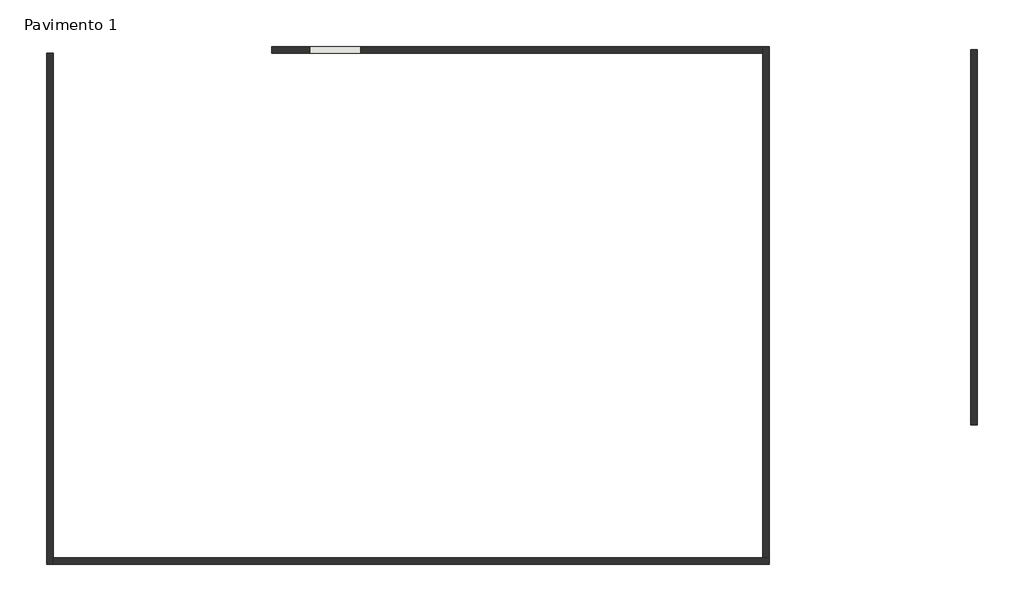
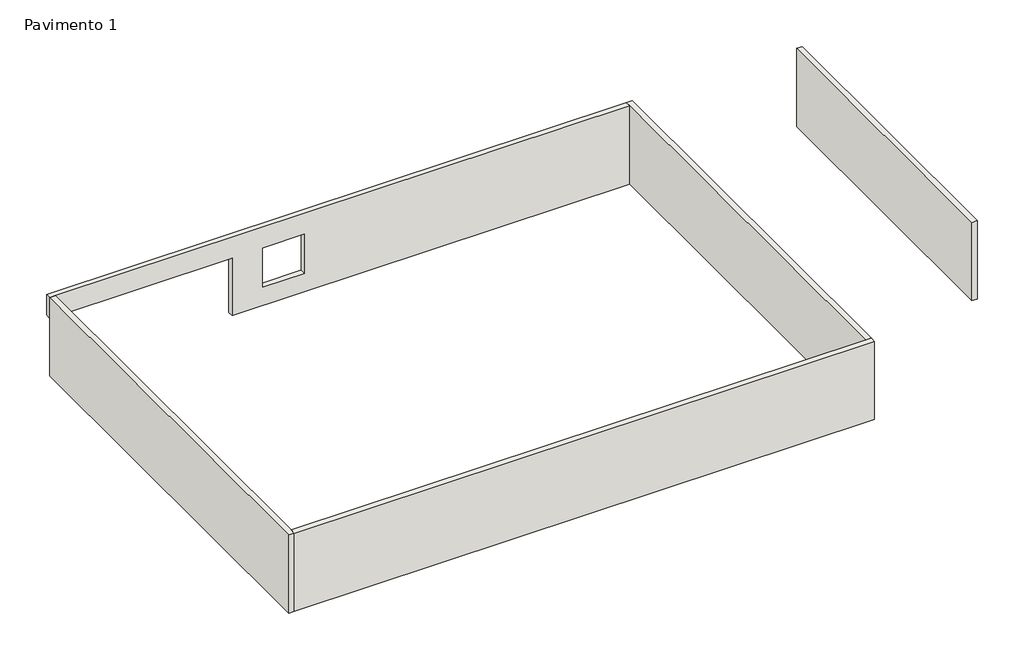
# One storey: 5 walls.
"""IFC4 building model written with IfcOpenShell, lengths in millimetres."""

from ifc_helpers import new_model, si_unit, origin, origin_with_axes, place, context, project, spatial, polyline, outline, extrude, faceted_brep, element, save

model = new_model("IFC4")

# Units and contexts
model_context = context("Model", 3, world=origin())
ifc_project = project(units=[si_unit("LENGTHUNIT", "METRE", prefix="MILLI")], contexts=[model_context])

# Site, building, storey
site = spatial("IfcSite", under=ifc_project)
building = spatial("IfcBuilding", under=site)
storey = spatial("IfcBuildingStorey", under=building, Name="Pavimento 1", Elevation=0.0)

# Walls
placement = place(None, origin())
element("IfcWall", 1, ObjectType=".Parede 020 cm", at=placement, inside=storey, context=model_context, shape_type="Brep", body=[
    faceted_brep([(-10926.104315, 4821.8769454, 2202.2712247), (-4326.104315, 4821.8769454, 2202.2712247), (-4326.104315, 4821.8769454, 0.0), (10073.895685, 4821.8769454, 0.0), (10073.895685, 4821.8769454, 3000.0), (-10726.104315, 4821.8769454, 3000.0), (-10926.104315, 4821.8769454, 3000.0), (-3207.6515293, 4821.8769454, 2202.2712247), (-1707.6515293, 4821.8769454, 2202.2712247), (-1707.6515293, 4821.8769454, 702.2712247), (-3207.6515293, 4821.8769454, 702.2712247), (-10926.104315, 5021.8769454, 2202.2712247), (-10926.104315, 5021.8769454, 3000.0), (10073.895685, 5021.8769454, 3000.0), (10073.895685, 5021.8769454, 0.0), (-4326.104315, 5021.8769454, 0.0), (-4326.104315, 5021.8769454, 2202.2712247), (-3207.6515293, 5021.8769454, 2202.2712247), (-3207.6515293, 5021.8769454, 702.2712247), (-1707.6515293, 5021.8769454, 702.2712247), (-1707.6515293, 5021.8769454, 2202.2712247)], [[[0, 1, 2, 3, 4, 5, 6], [7, 8, 9, 10]], [[11, 12, 13, 14, 15, 16], [17, 18, 19, 20]], [[0, 6, 12, 11]], [[4, 3, 14, 13]], [[3, 2, 15, 14]], [[6, 5, 4, 13, 12]], [[8, 7, 17, 20]], [[9, 8, 20, 19]], [[10, 9, 19, 18]], [[7, 10, 18, 17]], [[1, 0, 11, 16]], [[2, 1, 16, 15]]]),
])
element("IfcWall", 2, ObjectType=".Parede 020 cm", at=placement, inside=storey, context=model_context, shape_type="Brep", body=[
    faceted_brep([(-10726.104315, -10178.1230546, 0.0), (-10726.104315, -9978.1230546, 0.0), (-10726.104315, 4821.8769454, 0.0), (-10726.104315, 4821.8769454, 3000.0), (-10726.104315, -9978.1230546, 3000.0), (-10726.104315, -10178.1230546, 3000.0), (-10926.104315, -10178.1230546, 0.0), (-10926.104315, -10178.1230546, 3000.0), (-10926.104315, 4821.8769454, 3000.0), (-10926.104315, 4821.8769454, 2202.2712247), (-10926.104315, 4821.8769454, 0.0)], [[[0, 1, 2, 3, 4, 5]], [[6, 7, 8, 9, 10]], [[2, 1, 0, 6, 10]], [[5, 4, 3, 8, 7]], [[0, 5, 7, 6]], [[3, 2, 10, 9, 8]]]),
])
element("IfcWall", 3, ObjectType=".Parede 020 cm", at=placement, inside=storey, context=model_context, shape_type="Brep", body=[
    faceted_brep([(10273.895685, -9978.1230546, 0.0), (10073.895685, -9978.1230546, 0.0), (-10726.104315, -9978.1230546, 0.0), (-10726.104315, -9978.1230546, 3000.0), (10073.895685, -9978.1230546, 3000.0), (10273.895685, -9978.1230546, 3000.0), (10273.895685, -10178.1230546, 0.0), (10273.895685, -10178.1230546, 3000.0), (-10726.104315, -10178.1230546, 3000.0), (-10726.104315, -10178.1230546, 0.0)], [[[0, 1, 2, 3, 4, 5]], [[6, 7, 8, 9]], [[2, 1, 0, 6, 9]], [[5, 4, 3, 8, 7]], [[0, 5, 7, 6]], [[3, 2, 9, 8]]]),
])
element("IfcWall", 4, ObjectType=".Parede 020 cm", at=placement, inside=storey, context=model_context, shape_type="Brep", body=[
    faceted_brep([(10073.895685, 5021.8769454, 0.0), (10073.895685, 4821.8769454, 0.0), (10073.895685, -9978.1230546, 0.0), (10073.895685, -9978.1230546, 3000.0), (10073.895685, 4821.8769454, 3000.0), (10073.895685, 5021.8769454, 3000.0), (10273.895685, 5021.8769454, 0.0), (10273.895685, 5021.8769454, 3000.0), (10273.895685, -9978.1230546, 3000.0), (10273.895685, -9978.1230546, 0.0)], [[[0, 1, 2, 3, 4, 5]], [[6, 7, 8, 9]], [[2, 1, 0, 6, 9]], [[5, 4, 3, 8, 7]], [[0, 5, 7, 6]], [[3, 2, 9, 8]]]),
])
element("IfcWall", 5, ObjectType=".Parede 020 cm", at=placement, inside=storey, context=model_context, shape_type="SweptSolid", body=[
    extrude(outline(polyline([(16173.895685, -6078.1230546), (16173.895685, 4921.8769454), (16373.895685, 4921.8769454), (16373.895685, -6078.1230546), (16173.895685, -6078.1230546)])), origin_with_axes(), (0.0, 0.0, 1.0), 3000.0),
])

save(model, "model.ifc")

# Revit data of these elements
# Project information
#   Data de emissão do projeto = "Data de emissão"
#   Status do projeto = "Status do projeto"
#   Nome do cliente = "Proprietário"
#   Endereço do projeto = "Insira aqui o endereço"
#   Nome do projeto = "Nome do projeto"
#   Número do projeto = "0001"
# Type ".Parede 020 cm"
#   Layers, outside or top first: 0.01 m ".Tinta externa branco gelo" (function 4); 0.03 m ".Revestimento de concreto" (function 4); 0.12 m ".Tijolo 9 cm" (function 1); 0.03 m ".Revestimento de concreto" (function 4); 0.01 m ".Tinta externa branco gelo" (function 4)
# Element 1 (IfcWall, ".Parede 020 cm")
#   Top Offset = 0.00 m
#   Base Offset = 0.00 m
#   wall height = 3.00 m
#   Phase Created = Construção nova
#   Base Constraint = Pavimento 1
#   Top Constraint = Pavimento 2
#   Materials on its faces: "Material pré-definido de parede", ".Tinta bege"
# Element 2 (IfcWall, ".Parede 020 cm")
#   Top Offset = 0.00 m
#   Base Offset = 0.00 m
#   wall height = 3.00 m
#   Phase Created = Construção nova
#   Base Constraint = Pavimento 1
#   Top Constraint = Pavimento 2
#   Materials on its faces: ".Tinta bege", "Material pré-definido de parede"
# Element 3 (IfcWall, ".Parede 020 cm")
#   Top Offset = 0.00 m
#   Base Offset = 0.00 m
#   wall height = 3.00 m
#   Phase Created = Construção nova
#   Base Constraint = Pavimento 1
#   Top Constraint = Pavimento 2
#   Materials on its faces: ".Tinta bege", ".Tinta externa branco gelo", "Material pré-definido de parede"
# Element 4 (IfcWall, ".Parede 020 cm")
#   Top Offset = 0.00 m
#   Base Offset = 0.00 m
#   wall height = 3.00 m
#   Phase Created = Construção nova
#   Base Constraint = Pavimento 1
#   Top Constraint = Pavimento 2
#   Materials on its faces: ".Tinta bege", "Material pré-definido de parede", ".Tinta externa branco gelo"
# Element 5 (IfcWall, ".Parede 020 cm")
#   Top Offset = 0.00 m
#   Base Offset = 0.00 m
#   wall height = 3.00 m
#   Phase Created = Construção nova
#   Base Constraint = Pavimento 1
#   Top Constraint = Pavimento 2
#   Materials on its faces: ".Tinta externa branco gelo", ".Tinta bege", ".Pedras", "Material pré-definido de parede", ".Tijolo 9 cm"
# Materials
#   ".Tinta externa branco gelo": class "Genérico", colour RGB 210 210 210, transparency 0, Cost = 0
#   ".Revestimento de concreto": class "Genérico", colour RGB 120 120 120, transparency 0, Cost = 0
#   ".Tijolo 9 cm": class "Genérico", colour RGB 255 255 255, transparency 0, Cost = 0
#   "Material pré-definido de parede": class "Diversos", colour RGB 128 128 128, transparency 0, Cost = 0
#   ".Tinta bege": class "Genérico", colour RGB 245 245 245, transparency 0, Cost = 0
#   ".Pedras": class "Genérico", colour RGB 118 107 76, transparency 0, Cost = 0
